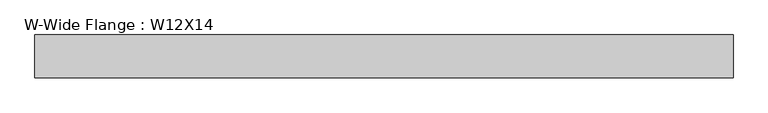
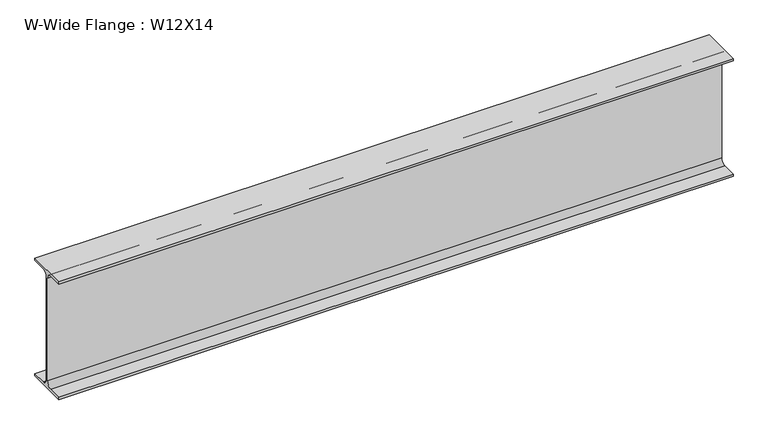
"""IFC4 building model written with IfcOpenShell, lengths in millimetres: beam geometry, W-Wide Flange : W12X14."""

from ifc_helpers import new_model, si_unit, point, frame, frame_2d, origin, place, context, project, spatial, polyline, circle_curve, trimmed, segment, composite_curve, outline, extrude, source, transform, mapped, element, save


def w_wide_flange_w12x14_21ad3ae7(model_context):
    return source(origin(), model_context, "Body", "SweptSolid", [
        extrude(outline(composite_curve([segment(polyline([(50.419, -145.415), (50.419, -151.13), (-50.419, -151.13), (-50.419, -145.415), (-15.875, -145.415)]), True, "CONTINUOUS"), segment(trimmed(circle_curve(frame_2d((-15.875, -132.08)), 13.335), [point((-15.875, -145.415))], [point((-2.54, -132.08))], True, "CARTESIAN"), True, "CONTINUOUS"), segment(polyline([(-2.54, -132.08), (-2.54, 132.08)]), True, "CONTINUOUS"), segment(trimmed(circle_curve(frame_2d((-15.875, 132.08)), 13.335), [point((-2.54, 132.08))], [point((-15.875, 145.415))], True, "CARTESIAN"), True, "CONTINUOUS"), segment(polyline([(-15.875, 145.415), (-50.419, 145.415), (-50.419, 151.13), (50.419, 151.13), (50.419, 145.415), (15.875, 145.415)]), True, "CONTINUOUS"), segment(trimmed(circle_curve(frame_2d((15.875, 132.08)), 13.335), [point((15.875, 145.415))], [point((2.54, 132.08))], True, "CARTESIAN"), True, "CONTINUOUS"), segment(polyline([(2.54, 132.08), (2.54, -132.08)]), True, "CONTINUOUS"), segment(trimmed(circle_curve(frame_2d((15.875, -132.08)), 13.335), [point((2.54, -132.08))], [point((15.875, -145.415))], True, "CARTESIAN"), True, "CONTINUOUS"), segment(polyline([(15.875, -145.415), (50.419, -145.415)]), True, "CONTINUOUS")], self_intersect=False)), frame((-812.927, 0.0, 0.0), z_axis=(1.0, 0.0, 0.0), x_axis=(0.0, 1.0, 0.0)), (0.0, 0.0, 1.0), 1638.427),
    ])


if __name__ == "__main__":
    model = new_model("IFC4")
    model_context = context("Model", 3, world=origin())
    ifc_project = project(units=[si_unit("LENGTHUNIT", "METRE", prefix="MILLI")], contexts=[model_context])
    site = spatial("IfcSite", under=ifc_project)
    building = spatial("IfcBuilding", under=site)
    placement = place(None, origin())
    w_wide_flange_w12x14_shape = w_wide_flange_w12x14_21ad3ae7(model_context)
    element("IfcBeam", 1, ObjectType="W-Wide Flange : W12X14", at=placement, inside=building, context=model_context, shape_type="MappedRepresentation", body=[
        mapped(w_wide_flange_w12x14_shape, transform((0.0, 0.0, 0.0), x_axis=(1.0, 0.0, 0.0), y_axis=(0.0, 1.0, 0.0), z_axis=(0.0, 0.0, 1.0))),
    ])
    save(model, "model.ifc")

# Revit data of these elements
# Type "W-Wide Flange : W12X14"
#   Assembly Code = "B10"
#   W = 14
#   Length [instance default] = 5' - 0"
#   bf = 0' - 3.97"
#   d = 0' - 11.9"
#   k = 0' - 0 3/4"
#   k2 = 0' - 0.525"
#   tf = 0' - 0.225"
#   tw = 0' - 0.2"
#   A = 0.0288889 SF
#   Structural Material [instance default] = Steel ASTM A992
# Element 1 (IfcBeam, "W-Wide Flange : W12X14")
#   Materials on its faces: "Steel ASTM A992"
# Materials
#   "Steel ASTM A992": class "Metal", colour RGB 199 199 199, transparency 0, Description = "Structural steel 50ksi", Cost = 0
